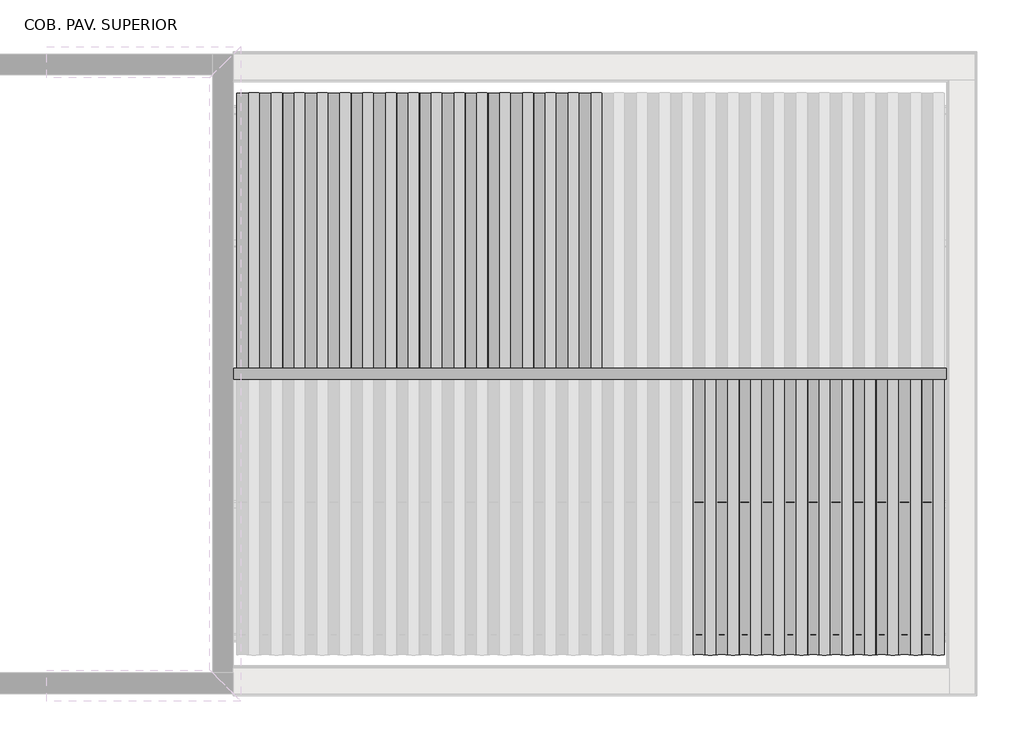
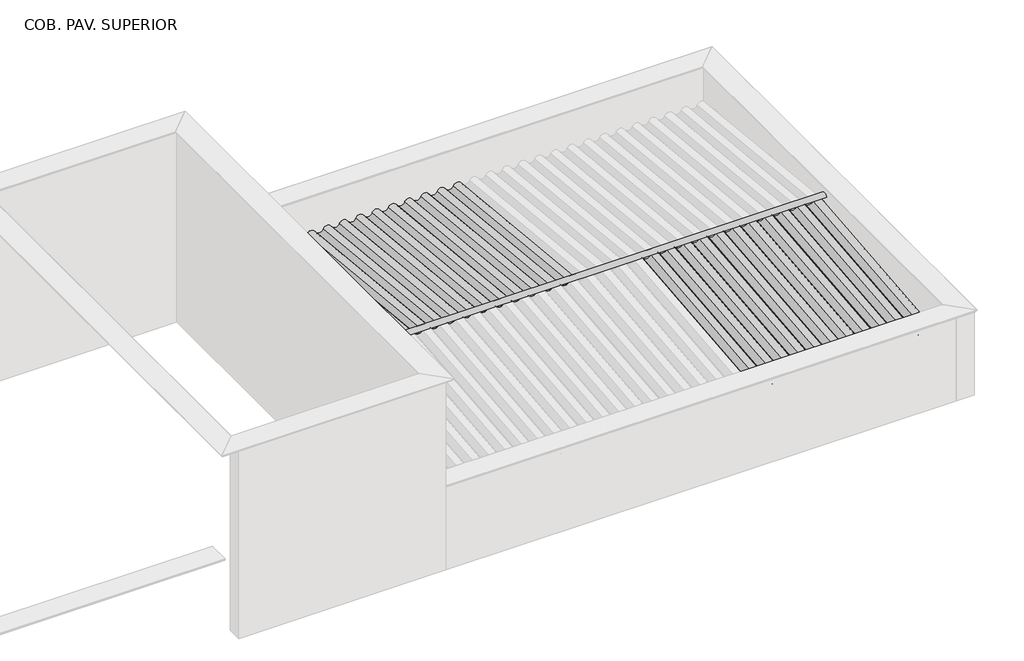
# One storey, part 6 of 7: 35 beams, 6 columns.
"""IFC4 building model written with IfcOpenShell, lengths in millimetres."""

import ifcopenshell
import ifcopenshell.guid

model = None  # the IFC model being written
_history = None  # IfcOwnerHistory: only IFC2X3 demands one
_inside = {}  # id of a spatial element -> (the spatial element, [elements in it])
_under = {}  # id of a project, library or spatial element -> (it, [spatial elements below it])
_declared = {}  # id of a project -> (the project, [libraries it declares])
_typed = {}  # id of a type object -> (the type object, [elements of that type])
_made_of = {}  # id of a material, layer set ... -> (it, [elements and type objects made of it])


def new_model(schema):
    """Start an empty IFC model of exactly this schema.

    Asked for "IFC4X3", IfcOpenShell would pick the latest addendum, in which some entities
    have other attributes; the version numbers below select the first issue.
    IFC2X3 requires an IfcOwnerHistory on every rooted entity: one is made here for all.
    """
    global model, _history
    if schema == "IFC4X3":
        model = ifcopenshell.file(schema_version=(4, 3, 0, 0))
    else:
        model = ifcopenshell.file(schema=schema)
    _inside.clear()
    _under.clear()
    _declared.clear()
    _typed.clear()
    _made_of.clear()
    _history = None
    if model.schema == "IFC2X3":
        org = make("IfcOrganization", Name="unknown")
        user = make(
            "IfcPersonAndOrganization",
            ThePerson=make("IfcPerson", FamilyName="unknown"),
            TheOrganization=org,
        )
        app = make(
            "IfcApplication",
            ApplicationDeveloper=org,
            Version="unknown",
            ApplicationFullName="unknown",
            ApplicationIdentifier="unknown",
        )
        _history = make(
            "IfcOwnerHistory",
            OwningUser=user,
            OwningApplication=app,
            ChangeAction="ADDED",
            CreationDate=0,
        )
    return model


def make(cls, **values):
    """One entity of the class cls with the attributes given. An attribute that is None is left unset."""
    return model.create_entity(
        cls, **{name: value for name, value in values.items() if value is not None}
    )


def rooted(cls, **values):
    """An entity with a GlobalId (a new one), such as an element, a storey or a relation."""
    return make(cls, GlobalId=ifcopenshell.guid.new(), OwnerHistory=_history, **values)


def si_unit(unit_type, name, prefix=None):
    """IfcSIUnit, for example si_unit("LENGTHUNIT", "METRE", prefix="MILLI")."""
    return make("IfcSIUnit", UnitType=unit_type, Prefix=prefix, Name=name)


def assignment(units):
    """IfcUnitAssignment: the units of a project."""
    return None if units is None else make("IfcUnitAssignment", Units=units)


def point(xyz):
    """IfcCartesianPoint."""
    return None if xyz is None else make("IfcCartesianPoint", Coordinates=xyz)


def direction(xyz):
    """IfcDirection."""
    return None if xyz is None else make("IfcDirection", DirectionRatios=xyz)


def frame(location, z_axis=None, x_axis=None):
    """IfcAxis2Placement3D, a coordinate frame: its origin and axes. An axis left out is left unset."""
    return make(
        "IfcAxis2Placement3D",
        Location=point(location),
        Axis=direction(z_axis),
        RefDirection=direction(x_axis),
    )


def frame_2d(location, x_axis=None):
    """IfcAxis2Placement2D, a coordinate frame in the plane: its origin and x axis."""
    return make(
        "IfcAxis2Placement2D", Location=point(location), RefDirection=direction(x_axis)
    )


def origin():
    """The frame at (0, 0, 0) with its axes left unset."""
    return frame((0.0, 0.0, 0.0))


def place(relative_to, where):
    """IfcLocalPlacement: puts the frame where relative to a parent placement (None: the world)."""
    return make(
        "IfcLocalPlacement", PlacementRelTo=relative_to, RelativePlacement=where
    )


def context(
    kind, dimensions, precision=None, world=None, true_north=None, identifier=None
):
    """IfcGeometricRepresentationContext, for example the 3D "Model" context."""
    return make(
        "IfcGeometricRepresentationContext",
        ContextIdentifier=identifier,
        ContextType=kind,
        CoordinateSpaceDimension=dimensions,
        Precision=precision,
        WorldCoordinateSystem=world,
        TrueNorth=true_north,
    )


def project(units=None, contexts=None):
    """IfcProject with its units and contexts."""
    return rooted(
        "IfcProject",
        Name="project",
        RepresentationContexts=contexts,
        UnitsInContext=assignment(units),
    )


def spatial(cls, under=None, at=None, **own):
    """A site, building, storey or space (cls), placed at a placement, below another one or the project."""
    s = rooted(cls, ObjectPlacement=at, **own)
    if under is not None:
        _under.setdefault(under.id(), (under, []))[1].append(s)
    return s


def polyline(points):
    """IfcPolyline through the points."""
    return make("IfcPolyline", Points=[point(p) for p in points])


def circle_curve(where, radius):
    """IfcCircle in the frame where."""
    return make("IfcCircle", Position=where, Radius=radius)


def trimmed(basis, trim1, trim2, sense, master):
    """IfcTrimmedCurve: the piece of a basis curve between two trims."""
    return make(
        "IfcTrimmedCurve",
        BasisCurve=basis,
        Trim1=trim1,
        Trim2=trim2,
        SenseAgreement=sense,
        MasterRepresentation=master,
    )


def segment(curve, same_sense, transition):
    """IfcCompositeCurveSegment."""
    return make(
        "IfcCompositeCurveSegment",
        Transition=transition,
        SameSense=same_sense,
        ParentCurve=curve,
    )


def composite_curve(segments, self_intersect=None):
    """IfcCompositeCurve: segments joined end to end."""
    return make("IfcCompositeCurve", Segments=segments, SelfIntersect=self_intersect)


def outline(outer, holes=None, kind="AREA"):
    """IfcArbitraryClosedProfileDef: a profile drawn as a closed curve; with holes, ...WithVoids."""
    if holes is None:
        return make("IfcArbitraryClosedProfileDef", ProfileType=kind, OuterCurve=outer)
    return make(
        "IfcArbitraryProfileDefWithVoids",
        ProfileType=kind,
        OuterCurve=outer,
        InnerCurves=holes,
    )


def extrude(swept, where, along, depth):
    """IfcExtrudedAreaSolid: the profile swept, set in the frame where, extruded along a direction by depth."""
    return make(
        "IfcExtrudedAreaSolid",
        SweptArea=swept,
        Position=where,
        ExtrudedDirection=direction(along),
        Depth=depth,
    )


def shape(context_of_items, identifier, shape_type, items):
    """IfcShapeRepresentation: the items that make up one representation, for example the "Body"."""
    return make(
        "IfcShapeRepresentation",
        ContextOfItems=context_of_items,
        RepresentationIdentifier=identifier,
        RepresentationType=shape_type,
        Items=items,
    )


def source(mapping_origin, context_of_items, identifier, shape_type, items):
    """IfcRepresentationMap: a shape defined once, which mapped items show again and again."""
    return make(
        "IfcRepresentationMap",
        MappingOrigin=mapping_origin,
        MappedRepresentation=shape(context_of_items, identifier, shape_type, items),
    )


def transform(
    local_origin,
    x_axis=None,
    y_axis=None,
    z_axis=None,
    scale=None,
    scale2=None,
    scale3=None,
    uniform=True,
):
    """IfcCartesianTransformationOperator3D, or its non-uniform kind. x_axis, y_axis, z_axis: its Axis1, 2, 3."""
    if uniform:
        return make(
            "IfcCartesianTransformationOperator3D",
            Axis1=direction(x_axis),
            Axis2=direction(y_axis),
            LocalOrigin=point(local_origin),
            Scale=scale,
            Axis3=direction(z_axis),
        )
    return make(
        "IfcCartesianTransformationOperator3DnonUniform",
        Axis1=direction(x_axis),
        Axis2=direction(y_axis),
        LocalOrigin=point(local_origin),
        Scale=scale,
        Axis3=direction(z_axis),
        Scale2=scale2,
        Scale3=scale3,
    )


def mapped(mapping_source, mapping_target):
    """IfcMappedItem: shows the shape of a source again, moved by a transform."""
    return make(
        "IfcMappedItem", MappingSource=mapping_source, MappingTarget=mapping_target
    )


def made_of(thing, what):
    """Note that an element or type object is made of a material, layer set ...; save() writes the relation."""
    if what is not None:
        _made_of.setdefault(what.id(), (what, []))[1].append(thing)
    return thing


def element(
    cls,
    number,
    at=None,
    inside=None,
    cuts=None,
    type_object=None,
    material=None,
    context=None,
    identifier="Body",
    shape_type=None,
    held_by="IfcProductDefinitionShape",
    body=None,
    shapes=None,
    **own,
):
    """One element of the class cls, such as IfcWall. Its Tag is "e" and its number.

    at: its placement. inside: the storey or other place that contains it. cuts: it is an
    opening in that element (IfcRelVoidsElement). A single representation is given by context,
    identifier, shape_type and body (its items); several are given by shapes. held_by: the class
    of the entity that holds the representations. save() writes the other relations.
    """
    e = rooted(cls, Tag="e%d" % number, ObjectPlacement=at, **own)
    if body is not None:
        shapes = [shape(context, identifier, shape_type, body)]
    if shapes is not None:
        e.Representation = make(held_by, Representations=shapes)
    if inside is not None:
        _inside.setdefault(inside.id(), (inside, []))[1].append(e)
    if cuts is not None:
        rooted(
            "IfcRelVoidsElement", RelatingBuildingElement=cuts, RelatedOpeningElement=e
        )
    if type_object is not None:
        _typed.setdefault(type_object.id(), (type_object, []))[1].append(e)
    return made_of(e, material)


def aggregate(whole, parts):
    """IfcRelAggregates: a whole, such as a stair, and the parts it consists of."""
    return rooted("IfcRelAggregates", RelatingObject=whole, RelatedObjects=parts)


def save(model, path):
    """Write the relations noted so far, then the file.

    IfcRelAggregates (storeys below a building ...), IfcRelContainedInSpatialStructure (elements
    in a storey), IfcRelDefinesByType, IfcRelAssociatesMaterial and IfcRelDeclares: one each for
    every whole, place, type object, material and project.
    """
    for whole, parts in _under.values():
        aggregate(whole, parts)
    for where, things in _inside.values():
        rooted(
            "IfcRelContainedInSpatialStructure",
            RelatedElements=things,
            RelatingStructure=where,
        )
    for kind, things in _typed.values():
        rooted("IfcRelDefinesByType", RelatedObjects=things, RelatingType=kind)
    for what, things in _made_of.values():
        rooted("IfcRelAssociatesMaterial", RelatedObjects=things, RelatingMaterial=what)
    for by, libraries in _declared.values():
        rooted("IfcRelDeclares", RelatingContext=by, RelatedDefinitions=libraries)
    model.write(path)


def cumeeira_telha_ondulada_fibrocimento_a8dbf5af(model_context):
    return source(origin(), model_context, "Body", "SweptSolid", [
        extrude(outline(composite_curve([segment(polyline([(58.3970135, 42.4437972), (53.9055884, 40.2467307)]), True, "CONTINUOUS"), segment(trimmed(circle_curve(frame_2d((-1.6029865, 13.0936483)), 61.7939461), [point((53.9055884, 40.2467307))], [point((-57.1115615, 40.2467307))], True, "CARTESIAN"), True, "CONTINUOUS"), segment(polyline([(-57.1115615, 40.2467307), (-61.6029865, 42.4437972)]), True, "CONTINUOUS"), segment(trimmed(circle_curve(frame_2d((-1.6029865, 13.0936483)), 66.7939461), [point((-61.6029865, 42.4437972))], [point((58.3970135, 42.4437972))], False, "CARTESIAN"), True, "CONTINUOUS")], self_intersect=False)), frame((-3970.0, 0.0, 0.0), z_axis=(1.0, 0.0, 0.0), x_axis=(0.0, 1.0, 0.0)), (0.0, 0.0, 1.0), 7940.0),
    ])


def viga_cumeeira_6x16cm_8fcfcc43(model_context):
    return source(origin(), model_context, "Body", "SweptSolid", [
        extrude(outline(polyline([(3822.5, 30.0), (3822.5, -30.0), (-3822.5, -30.0), (-3822.5, 30.0), (3822.5, 30.0)])), frame((0.0, 0.0, -80.0), z_axis=(0.0, 0.0, 1.0), x_axis=(1.0, 0.0, 0.0)), (0.0, 0.0, 1.0), 160.0),
    ])


def column_d505325c(model_context):
    return source(origin(), model_context, "Body", "SweptSolid", [
        extrude(outline(polyline([(30.0, 80.0), (30.0, -80.0), (-30.0, -80.0), (-30.0, 80.0), (30.0, 80.0)])), frame((0.0, 0.0, 6710.0), z_axis=(0.0, 0.0, 1.0), x_axis=(1.0, 0.0, 0.0)), (0.0, 0.0, 1.0), 750.0),
    ])


def column_4db371bd(model_context):
    return source(origin(), model_context, "Body", "SweptSolid", [
        extrude(outline(polyline([(30.0, 80.0), (30.0, -80.0), (-30.0, -80.0), (-30.0, 80.0), (30.0, 80.0)])), frame((0.0, 0.0, 6710.0), z_axis=(0.0, 0.0, 1.0), x_axis=(1.0, 0.0, 0.0)), (0.0, 0.0, 1.0), 660.0),
    ])


model = new_model("IFC4")

# Units and contexts
model_context = context("Model", 3, world=origin())
ifc_project = project(units=[si_unit("LENGTHUNIT", "METRE", prefix="MILLI")], contexts=[model_context])

# Site, building, storey
site = spatial("IfcSite", under=ifc_project)
building = spatial("IfcBuilding", under=site)
storey = spatial("IfcBuildingStorey", under=building, Name="COB. PAV. SUPERIOR", Elevation=6650.0)

# Beams
placement = place(None, origin())
element("IfcBeam", 1, ObjectType="Madeira de lei : Berço 6x12cm", at=placement, inside=storey, context=model_context, shape_type="SweptSolid", body=[
    extrude(outline(polyline([(5090.718693, -7711.5607799), (5090.718693, -7831.5607799), (3090.718693, -7831.5607799), (3090.718693, -7711.5607799), (5090.718693, -7711.5607799)])), frame((0.0, 0.0, 6650.0), z_axis=(0.0, 0.0, 1.0), x_axis=(1.0, 0.0, 0.0)), (0.0, 0.0, 1.0), 60.0),
])
element("IfcBeam", 2, ObjectType="Madeira de lei : Berço 6x12cm", at=placement, inside=storey, context=model_context, shape_type="SweptSolid", body=[
    extrude(outline(polyline([(7090.718693, -7711.5607799), (7090.718693, -7831.5607799), (5090.718693, -7831.5607799), (5090.718693, -7711.5607799), (7090.718693, -7711.5607799)])), frame((0.0, 0.0, 6650.0), z_axis=(0.0, 0.0, 1.0), x_axis=(1.0, 0.0, 0.0)), (0.0, 0.0, 1.0), 60.0),
])
element("IfcBeam", 3, ObjectType="Madeira de lei : Berço 6x12cm", at=placement, inside=storey, context=model_context, shape_type="SweptSolid", body=[
    extrude(outline(polyline([(5089.7186924, -6319.8711004), (5089.7186924, -6439.8711004), (3089.718693, -6439.8711004), (3089.718693, -6319.8711004), (5089.7186924, -6319.8711004)])), frame((0.0, 0.0, 6650.0), z_axis=(0.0, 0.0, 1.0), x_axis=(1.0, 0.0, 0.0)), (0.0, 0.0, 1.0), 60.0),
])
element("IfcBeam", 4, ObjectType="Madeira de lei : Berço 6x12cm", at=placement, inside=storey, context=model_context, shape_type="SweptSolid", body=[
    extrude(outline(polyline([(7089.7186924, -6319.8711004), (7089.7186924, -6439.8711004), (5089.7186936, -6439.8711004), (5089.7186936, -6319.8711004), (7089.7186924, -6319.8711004)])), frame((0.0, 0.0, 6650.0), z_axis=(0.0, 0.0, 1.0), x_axis=(1.0, 0.0, 0.0)), (0.0, 0.0, 1.0), 60.0),
])
element("IfcBeam", 5, ObjectType="Madeira de lei : Berço 6x12cm", at=placement, inside=storey, context=model_context, shape_type="SweptSolid", body=[
    extrude(outline(polyline([(9089.718693, -9101.268869), (9089.718693, -9221.268869), (7089.718693, -9221.268869), (7089.718693, -9101.268869), (9089.718693, -9101.268869)])), frame((0.0, 0.0, 6650.0), z_axis=(0.0, 0.0, 1.0), x_axis=(1.0, 0.0, 0.0)), (0.0, 0.0, 1.0), 60.0),
])
element("IfcBeam", 6, ObjectType="Madeira de lei : Berço 6x12cm", at=placement, inside=storey, context=model_context, shape_type="SweptSolid", body=[
    extrude(outline(polyline([(10709.718693, -9101.268869), (10709.718693, -9221.268869), (9089.718693, -9221.268869), (9089.718693, -9101.268869), (10709.718693, -9101.268869)])), frame((0.0, 0.0, 6650.0), z_axis=(0.0, 0.0, 1.0), x_axis=(1.0, 0.0, 0.0)), (0.0, 0.0, 1.0), 60.0),
])
cumeeira_telha_ondulada_fibrocimento_shape = cumeeira_telha_ondulada_fibrocimento_a8dbf5af(model_context)
element("IfcBeam", 7, ObjectType="Cumeeira Telha Ondulada : Fibrocimento", at=placement, inside=storey, context=model_context, shape_type="MappedRepresentation", body=[
    mapped(cumeeira_telha_ondulada_fibrocimento_shape, transform((7061.718693, -7771.5607799, 7660.6251229), x_axis=(-1.0, 0.0, 0.0), y_axis=(0.0, -1.0, 0.0), z_axis=(0.0, 0.0, 1.0))),
])
element("IfcBeam", 8, ObjectType="Telha Ondulada : Fibrocimento", at=placement, inside=storey, context=model_context, shape_type="SweptSolid", body=[
    extrude(outline(composite_curve([segment(trimmed(circle_curve(frame_2d((-58.7002978, -53.2060539)), 66.7939461), [point((-29.3501489, 6.7939461))], [point((-29.3501489, -113.2060539))], False, "CARTESIAN"), True, "CONTINUOUS"), segment(polyline([(-29.3501489, -113.2060539), (-31.5472154, -108.7146289)]), True, "CONTINUOUS"), segment(trimmed(circle_curve(frame_2d((-58.7002978, -53.2060539)), 61.7939461), [point((-31.5472154, -108.7146289))], [point((-31.5472154, 2.3025211))], True, "CARTESIAN"), True, "CONTINUOUS"), segment(trimmed(circle_curve(frame_2d((0.0, 66.7939461)), 71.7939461), [point((-31.5472154, 2.3025211))], [point((-31.5472154, 131.2853711))], False, "CARTESIAN"), True, "CONTINUOUS"), segment(polyline([(-31.5472154, 131.2853711), (-29.3501489, 126.7939461)]), True, "CONTINUOUS"), segment(trimmed(circle_curve(frame_2d((0.0, 66.7939461)), 66.7939461), [point((-29.3501489, 126.7939461))], [point((-29.3501489, 6.7939461))], True, "CARTESIAN"), True, "CONTINUOUS")], self_intersect=False)), frame((3256.1156257, -4759.1621575, 7394.5315886), z_axis=(0.0, -0.9950371902099893, 0.09950371902099778), x_axis=(0.0, 0.09950371902099778, 0.9950371902099893)), (0.0, 0.0, 1.0), 3017.2387654),
])
element("IfcBeam", 9, ObjectType="Telha Ondulada : Fibrocimento", at=placement, inside=storey, context=model_context, shape_type="SweptSolid", body=[
    extrude(outline(composite_curve([segment(trimmed(circle_curve(frame_2d((-58.7002978, -53.2060539)), 66.7939461), [point((-29.3501489, 6.7939461))], [point((-29.3501489, -113.2060539))], False, "CARTESIAN"), True, "CONTINUOUS"), segment(polyline([(-29.3501489, -113.2060539), (-31.5472154, -108.7146289)]), True, "CONTINUOUS"), segment(trimmed(circle_curve(frame_2d((-58.7002978, -53.2060539)), 61.7939461), [point((-31.5472154, -108.7146289))], [point((-31.5472154, 2.3025211))], True, "CARTESIAN"), True, "CONTINUOUS"), segment(trimmed(circle_curve(frame_2d((0.0, 66.7939461)), 71.7939461), [point((-31.5472154, 2.3025211))], [point((-31.5472154, 131.2853711))], False, "CARTESIAN"), True, "CONTINUOUS"), segment(polyline([(-31.5472154, 131.2853711), (-29.3501489, 126.7939461)]), True, "CONTINUOUS"), segment(trimmed(circle_curve(frame_2d((0.0, 66.7939461)), 66.7939461), [point((-29.3501489, 126.7939461))], [point((-29.3501489, 6.7939461))], True, "CARTESIAN"), True, "CONTINUOUS")], self_intersect=False)), frame((3500.6156257, -4759.1621575, 7394.5315886), z_axis=(0.0, -0.9950371902099893, 0.09950371902099778), x_axis=(0.0, 0.09950371902099778, 0.9950371902099893)), (0.0, 0.0, 1.0), 3017.2387654),
])
element("IfcBeam", 10, ObjectType="Telha Ondulada : Fibrocimento", at=placement, inside=storey, context=model_context, shape_type="SweptSolid", body=[
    extrude(outline(composite_curve([segment(trimmed(circle_curve(frame_2d((-58.7002978, -53.2060539)), 66.7939461), [point((-29.3501489, 6.7939461))], [point((-29.3501489, -113.2060539))], False, "CARTESIAN"), True, "CONTINUOUS"), segment(polyline([(-29.3501489, -113.2060539), (-31.5472154, -108.7146289)]), True, "CONTINUOUS"), segment(trimmed(circle_curve(frame_2d((-58.7002978, -53.2060539)), 61.7939461), [point((-31.5472154, -108.7146289))], [point((-31.5472154, 2.3025211))], True, "CARTESIAN"), True, "CONTINUOUS"), segment(trimmed(circle_curve(frame_2d((0.0, 66.7939461)), 71.7939461), [point((-31.5472154, 2.3025211))], [point((-31.5472154, 131.2853711))], False, "CARTESIAN"), True, "CONTINUOUS"), segment(polyline([(-31.5472154, 131.2853711), (-29.3501489, 126.7939461)]), True, "CONTINUOUS"), segment(trimmed(circle_curve(frame_2d((0.0, 66.7939461)), 66.7939461), [point((-29.3501489, 126.7939461))], [point((-29.3501489, 6.7939461))], True, "CARTESIAN"), True, "CONTINUOUS")], self_intersect=False)), frame((3745.1156257, -4759.1621575, 7394.5315886), z_axis=(0.0, -0.9950371902099893, 0.09950371902099776), x_axis=(0.0, 0.09950371902099776, 0.9950371902099893)), (0.0, 0.0, 1.0), 3017.2387654),
])
element("IfcBeam", 11, ObjectType="Telha Ondulada : Fibrocimento", at=placement, inside=storey, context=model_context, shape_type="SweptSolid", body=[
    extrude(outline(composite_curve([segment(trimmed(circle_curve(frame_2d((-58.7002978, -53.2060539)), 66.7939461), [point((-29.3501489, 6.7939461))], [point((-29.3501489, -113.2060539))], False, "CARTESIAN"), True, "CONTINUOUS"), segment(polyline([(-29.3501489, -113.2060539), (-31.5472154, -108.7146289)]), True, "CONTINUOUS"), segment(trimmed(circle_curve(frame_2d((-58.7002978, -53.2060539)), 61.7939461), [point((-31.5472154, -108.7146289))], [point((-31.5472154, 2.3025211))], True, "CARTESIAN"), True, "CONTINUOUS"), segment(trimmed(circle_curve(frame_2d((0.0, 66.7939461)), 71.7939461), [point((-31.5472154, 2.3025211))], [point((-31.5472154, 131.2853711))], False, "CARTESIAN"), True, "CONTINUOUS"), segment(polyline([(-31.5472154, 131.2853711), (-29.3501489, 126.7939461)]), True, "CONTINUOUS"), segment(trimmed(circle_curve(frame_2d((0.0, 66.7939461)), 66.7939461), [point((-29.3501489, 126.7939461))], [point((-29.3501489, 6.7939461))], True, "CARTESIAN"), True, "CONTINUOUS")], self_intersect=False)), frame((3989.6156257, -4759.1621575, 7394.5315886), z_axis=(0.0, -0.9950371902099893, 0.09950371902099776), x_axis=(0.0, 0.09950371902099776, 0.9950371902099893)), (0.0, 0.0, 1.0), 3017.2387654),
])
element("IfcBeam", 12, ObjectType="Telha Ondulada : Fibrocimento", at=placement, inside=storey, context=model_context, shape_type="SweptSolid", body=[
    extrude(outline(composite_curve([segment(trimmed(circle_curve(frame_2d((-58.7002978, -53.2060539)), 66.7939461), [point((-29.3501489, 6.7939461))], [point((-29.3501489, -113.2060539))], False, "CARTESIAN"), True, "CONTINUOUS"), segment(polyline([(-29.3501489, -113.2060539), (-31.5472154, -108.7146289)]), True, "CONTINUOUS"), segment(trimmed(circle_curve(frame_2d((-58.7002978, -53.2060539)), 61.7939461), [point((-31.5472154, -108.7146289))], [point((-31.5472154, 2.3025211))], True, "CARTESIAN"), True, "CONTINUOUS"), segment(trimmed(circle_curve(frame_2d((0.0, 66.7939461)), 71.7939461), [point((-31.5472154, 2.3025211))], [point((-31.5472154, 131.2853711))], False, "CARTESIAN"), True, "CONTINUOUS"), segment(polyline([(-31.5472154, 131.2853711), (-29.3501489, 126.7939461)]), True, "CONTINUOUS"), segment(trimmed(circle_curve(frame_2d((0.0, 66.7939461)), 66.7939461), [point((-29.3501489, 126.7939461))], [point((-29.3501489, 6.7939461))], True, "CARTESIAN"), True, "CONTINUOUS")], self_intersect=False)), frame((4234.1156257, -4759.1621575, 7394.5315886), z_axis=(0.0, -0.9950371902099893, 0.09950371902099775), x_axis=(0.0, 0.09950371902099775, 0.9950371902099893)), (0.0, 0.0, 1.0), 3017.2387654),
])
element("IfcBeam", 13, ObjectType="Telha Ondulada : Fibrocimento", at=placement, inside=storey, context=model_context, shape_type="SweptSolid", body=[
    extrude(outline(composite_curve([segment(trimmed(circle_curve(frame_2d((-58.7002978, -53.2060539)), 66.7939461), [point((-29.3501489, 6.7939461))], [point((-29.3501489, -113.2060539))], False, "CARTESIAN"), True, "CONTINUOUS"), segment(polyline([(-29.3501489, -113.2060539), (-31.5472154, -108.7146289)]), True, "CONTINUOUS"), segment(trimmed(circle_curve(frame_2d((-58.7002978, -53.2060539)), 61.7939461), [point((-31.5472154, -108.7146289))], [point((-31.5472154, 2.3025211))], True, "CARTESIAN"), True, "CONTINUOUS"), segment(trimmed(circle_curve(frame_2d((0.0, 66.7939461)), 71.7939461), [point((-31.5472154, 2.3025211))], [point((-31.5472154, 131.2853711))], False, "CARTESIAN"), True, "CONTINUOUS"), segment(polyline([(-31.5472154, 131.2853711), (-29.3501489, 126.7939461)]), True, "CONTINUOUS"), segment(trimmed(circle_curve(frame_2d((0.0, 66.7939461)), 66.7939461), [point((-29.3501489, 126.7939461))], [point((-29.3501489, 6.7939461))], True, "CARTESIAN"), True, "CONTINUOUS")], self_intersect=False)), frame((4478.6156257, -4759.1621575, 7394.5315886), z_axis=(0.0, -0.9950371902099893, 0.09950371902099778), x_axis=(0.0, 0.09950371902099778, 0.9950371902099893)), (0.0, 0.0, 1.0), 3017.2387654),
])
element("IfcBeam", 14, ObjectType="Telha Ondulada : Fibrocimento", at=placement, inside=storey, context=model_context, shape_type="SweptSolid", body=[
    extrude(outline(composite_curve([segment(trimmed(circle_curve(frame_2d((-58.7002978, -53.2060539)), 66.7939461), [point((-29.3501489, 6.7939461))], [point((-29.3501489, -113.2060539))], False, "CARTESIAN"), True, "CONTINUOUS"), segment(polyline([(-29.3501489, -113.2060539), (-31.5472154, -108.7146289)]), True, "CONTINUOUS"), segment(trimmed(circle_curve(frame_2d((-58.7002978, -53.2060539)), 61.7939461), [point((-31.5472154, -108.7146289))], [point((-31.5472154, 2.3025211))], True, "CARTESIAN"), True, "CONTINUOUS"), segment(trimmed(circle_curve(frame_2d((0.0, 66.7939461)), 71.7939461), [point((-31.5472154, 2.3025211))], [point((-31.5472154, 131.2853711))], False, "CARTESIAN"), True, "CONTINUOUS"), segment(polyline([(-31.5472154, 131.2853711), (-29.3501489, 126.7939461)]), True, "CONTINUOUS"), segment(trimmed(circle_curve(frame_2d((0.0, 66.7939461)), 66.7939461), [point((-29.3501489, 126.7939461))], [point((-29.3501489, 6.7939461))], True, "CARTESIAN"), True, "CONTINUOUS")], self_intersect=False)), frame((4723.1156257, -4759.1621575, 7394.5315886), z_axis=(0.0, -0.9950371902099893, 0.09950371902099776), x_axis=(0.0, 0.09950371902099776, 0.9950371902099893)), (0.0, 0.0, 1.0), 3017.2387654),
])
element("IfcBeam", 15, ObjectType="Telha Ondulada : Fibrocimento", at=placement, inside=storey, context=model_context, shape_type="SweptSolid", body=[
    extrude(outline(composite_curve([segment(trimmed(circle_curve(frame_2d((-58.7002978, -53.2060539)), 66.7939461), [point((-29.3501489, 6.7939461))], [point((-29.3501489, -113.2060539))], False, "CARTESIAN"), True, "CONTINUOUS"), segment(polyline([(-29.3501489, -113.2060539), (-31.5472154, -108.7146289)]), True, "CONTINUOUS"), segment(trimmed(circle_curve(frame_2d((-58.7002978, -53.2060539)), 61.7939461), [point((-31.5472154, -108.7146289))], [point((-31.5472154, 2.3025211))], True, "CARTESIAN"), True, "CONTINUOUS"), segment(trimmed(circle_curve(frame_2d((0.0, 66.7939461)), 71.7939461), [point((-31.5472154, 2.3025211))], [point((-31.5472154, 131.2853711))], False, "CARTESIAN"), True, "CONTINUOUS"), segment(polyline([(-31.5472154, 131.2853711), (-29.3501489, 126.7939461)]), True, "CONTINUOUS"), segment(trimmed(circle_curve(frame_2d((0.0, 66.7939461)), 66.7939461), [point((-29.3501489, 126.7939461))], [point((-29.3501489, 6.7939461))], True, "CARTESIAN"), True, "CONTINUOUS")], self_intersect=False)), frame((4967.6156257, -4759.1621575, 7394.5315886), z_axis=(0.0, -0.9950371902099893, 0.09950371902099775), x_axis=(0.0, 0.09950371902099775, 0.9950371902099893)), (0.0, 0.0, 1.0), 3017.2387654),
])
element("IfcBeam", 16, ObjectType="Telha Ondulada : Fibrocimento", at=placement, inside=storey, context=model_context, shape_type="SweptSolid", body=[
    extrude(outline(composite_curve([segment(trimmed(circle_curve(frame_2d((-58.7002978, -53.2060539)), 66.7939461), [point((-29.3501489, 6.7939461))], [point((-29.3501489, -113.2060539))], False, "CARTESIAN"), True, "CONTINUOUS"), segment(polyline([(-29.3501489, -113.2060539), (-31.5472154, -108.7146289)]), True, "CONTINUOUS"), segment(trimmed(circle_curve(frame_2d((-58.7002978, -53.2060539)), 61.7939461), [point((-31.5472154, -108.7146289))], [point((-31.5472154, 2.3025211))], True, "CARTESIAN"), True, "CONTINUOUS"), segment(trimmed(circle_curve(frame_2d((0.0, 66.7939461)), 71.7939461), [point((-31.5472154, 2.3025211))], [point((-31.5472154, 131.2853711))], False, "CARTESIAN"), True, "CONTINUOUS"), segment(polyline([(-31.5472154, 131.2853711), (-29.3501489, 126.7939461)]), True, "CONTINUOUS"), segment(trimmed(circle_curve(frame_2d((0.0, 66.7939461)), 66.7939461), [point((-29.3501489, 126.7939461))], [point((-29.3501489, 6.7939461))], True, "CARTESIAN"), True, "CONTINUOUS")], self_intersect=False)), frame((5212.1156257, -4759.1621575, 7394.5315886), z_axis=(0.0, -0.9950371902099893, 0.09950371902099778), x_axis=(0.0, 0.09950371902099778, 0.9950371902099893)), (0.0, 0.0, 1.0), 3017.2387654),
])
element("IfcBeam", 17, ObjectType="Telha Ondulada : Fibrocimento", at=placement, inside=storey, context=model_context, shape_type="SweptSolid", body=[
    extrude(outline(composite_curve([segment(trimmed(circle_curve(frame_2d((-58.7002978, -53.2060539)), 66.7939461), [point((-29.3501489, 6.7939461))], [point((-29.3501489, -113.2060539))], False, "CARTESIAN"), True, "CONTINUOUS"), segment(polyline([(-29.3501489, -113.2060539), (-31.5472154, -108.7146289)]), True, "CONTINUOUS"), segment(trimmed(circle_curve(frame_2d((-58.7002978, -53.2060539)), 61.7939461), [point((-31.5472154, -108.7146289))], [point((-31.5472154, 2.3025211))], True, "CARTESIAN"), True, "CONTINUOUS"), segment(trimmed(circle_curve(frame_2d((0.0, 66.7939461)), 71.7939461), [point((-31.5472154, 2.3025211))], [point((-31.5472154, 131.2853711))], False, "CARTESIAN"), True, "CONTINUOUS"), segment(polyline([(-31.5472154, 131.2853711), (-29.3501489, 126.7939461)]), True, "CONTINUOUS"), segment(trimmed(circle_curve(frame_2d((0.0, 66.7939461)), 66.7939461), [point((-29.3501489, 126.7939461))], [point((-29.3501489, 6.7939461))], True, "CARTESIAN"), True, "CONTINUOUS")], self_intersect=False)), frame((5456.6156257, -4759.1621575, 7394.5315886), z_axis=(0.0, -0.9950371902099893, 0.09950371902099776), x_axis=(0.0, 0.09950371902099776, 0.9950371902099893)), (0.0, 0.0, 1.0), 3017.2387654),
])
element("IfcBeam", 18, ObjectType="Telha Ondulada : Fibrocimento", at=placement, inside=storey, context=model_context, shape_type="SweptSolid", body=[
    extrude(outline(composite_curve([segment(trimmed(circle_curve(frame_2d((-58.7002978, -53.2060539)), 66.7939461), [point((-29.3501489, 6.7939461))], [point((-29.3501489, -113.2060539))], False, "CARTESIAN"), True, "CONTINUOUS"), segment(polyline([(-29.3501489, -113.2060539), (-31.5472154, -108.7146289)]), True, "CONTINUOUS"), segment(trimmed(circle_curve(frame_2d((-58.7002978, -53.2060539)), 61.7939461), [point((-31.5472154, -108.7146289))], [point((-31.5472154, 2.3025211))], True, "CARTESIAN"), True, "CONTINUOUS"), segment(trimmed(circle_curve(frame_2d((0.0, 66.7939461)), 71.7939461), [point((-31.5472154, 2.3025211))], [point((-31.5472154, 131.2853711))], False, "CARTESIAN"), True, "CONTINUOUS"), segment(polyline([(-31.5472154, 131.2853711), (-29.3501489, 126.7939461)]), True, "CONTINUOUS"), segment(trimmed(circle_curve(frame_2d((0.0, 66.7939461)), 66.7939461), [point((-29.3501489, 126.7939461))], [point((-29.3501489, 6.7939461))], True, "CARTESIAN"), True, "CONTINUOUS")], self_intersect=False)), frame((5701.1156257, -4759.1621575, 7394.5315886), z_axis=(0.0, -0.9950371902099893, 0.09950371902099776), x_axis=(0.0, 0.09950371902099776, 0.9950371902099893)), (0.0, 0.0, 1.0), 3017.2387654),
])
element("IfcBeam", 19, ObjectType="Telha Ondulada : Fibrocimento", at=placement, inside=storey, context=model_context, shape_type="SweptSolid", body=[
    extrude(outline(composite_curve([segment(trimmed(circle_curve(frame_2d((-58.7002978, -53.2060539)), 66.7939461), [point((-29.3501489, 6.7939461))], [point((-29.3501489, -113.2060539))], False, "CARTESIAN"), True, "CONTINUOUS"), segment(polyline([(-29.3501489, -113.2060539), (-31.5472154, -108.7146289)]), True, "CONTINUOUS"), segment(trimmed(circle_curve(frame_2d((-58.7002978, -53.2060539)), 61.7939461), [point((-31.5472154, -108.7146289))], [point((-31.5472154, 2.3025211))], True, "CARTESIAN"), True, "CONTINUOUS"), segment(trimmed(circle_curve(frame_2d((0.0, 66.7939461)), 71.7939461), [point((-31.5472154, 2.3025211))], [point((-31.5472154, 131.2853711))], False, "CARTESIAN"), True, "CONTINUOUS"), segment(polyline([(-31.5472154, 131.2853711), (-29.3501489, 126.7939461)]), True, "CONTINUOUS"), segment(trimmed(circle_curve(frame_2d((0.0, 66.7939461)), 66.7939461), [point((-29.3501489, 126.7939461))], [point((-29.3501489, 6.7939461))], True, "CARTESIAN"), True, "CONTINUOUS")], self_intersect=False)), frame((5945.6156257, -4759.1621575, 7394.5315886), z_axis=(0.0, -0.9950371902099893, 0.09950371902099778), x_axis=(0.0, 0.09950371902099778, 0.9950371902099893)), (0.0, 0.0, 1.0), 3017.2387654),
])
element("IfcBeam", 20, ObjectType="Telha Ondulada : Fibrocimento", at=placement, inside=storey, context=model_context, shape_type="SweptSolid", body=[
    extrude(outline(composite_curve([segment(trimmed(circle_curve(frame_2d((-58.7002978, -53.2060539)), 66.7939461), [point((-29.3501489, 6.7939461))], [point((-29.3501489, -113.2060539))], False, "CARTESIAN"), True, "CONTINUOUS"), segment(polyline([(-29.3501489, -113.2060539), (-31.5472154, -108.7146289)]), True, "CONTINUOUS"), segment(trimmed(circle_curve(frame_2d((-58.7002978, -53.2060539)), 61.7939461), [point((-31.5472154, -108.7146289))], [point((-31.5472154, 2.3025211))], True, "CARTESIAN"), True, "CONTINUOUS"), segment(trimmed(circle_curve(frame_2d((0.0, 66.7939461)), 71.7939461), [point((-31.5472154, 2.3025211))], [point((-31.5472154, 131.2853711))], False, "CARTESIAN"), True, "CONTINUOUS"), segment(polyline([(-31.5472154, 131.2853711), (-29.3501489, 126.7939461)]), True, "CONTINUOUS"), segment(trimmed(circle_curve(frame_2d((0.0, 66.7939461)), 66.7939461), [point((-29.3501489, 126.7939461))], [point((-29.3501489, 6.7939461))], True, "CARTESIAN"), True, "CONTINUOUS")], self_intersect=False)), frame((6190.1156257, -4759.1621575, 7394.5315886), z_axis=(0.0, -0.9950371902099893, 0.09950371902099778), x_axis=(0.0, 0.09950371902099778, 0.9950371902099893)), (0.0, 0.0, 1.0), 3017.2387654),
])
element("IfcBeam", 21, ObjectType="Telha Ondulada : Fibrocimento", at=placement, inside=storey, context=model_context, shape_type="SweptSolid", body=[
    extrude(outline(composite_curve([segment(trimmed(circle_curve(frame_2d((-58.7002978, -53.2060539)), 66.7939461), [point((-29.3501489, 6.7939461))], [point((-29.3501489, -113.2060539))], False, "CARTESIAN"), True, "CONTINUOUS"), segment(polyline([(-29.3501489, -113.2060539), (-31.5472154, -108.7146289)]), True, "CONTINUOUS"), segment(trimmed(circle_curve(frame_2d((-58.7002978, -53.2060539)), 61.7939461), [point((-31.5472154, -108.7146289))], [point((-31.5472154, 2.3025211))], True, "CARTESIAN"), True, "CONTINUOUS"), segment(trimmed(circle_curve(frame_2d((0.0, 66.7939461)), 71.7939461), [point((-31.5472154, 2.3025211))], [point((-31.5472154, 131.2853711))], False, "CARTESIAN"), True, "CONTINUOUS"), segment(polyline([(-31.5472154, 131.2853711), (-29.3501489, 126.7939461)]), True, "CONTINUOUS"), segment(trimmed(circle_curve(frame_2d((0.0, 66.7939461)), 66.7939461), [point((-29.3501489, 126.7939461))], [point((-29.3501489, 6.7939461))], True, "CARTESIAN"), True, "CONTINUOUS")], self_intersect=False)), frame((6434.6156257, -4759.1621575, 7394.5315886), z_axis=(0.0, -0.9950371902099893, 0.09950371902099776), x_axis=(0.0, 0.09950371902099776, 0.9950371902099893)), (0.0, 0.0, 1.0), 3017.2387654),
])
element("IfcBeam", 22, ObjectType="Telha Ondulada : Fibrocimento", at=placement, inside=storey, context=model_context, shape_type="SweptSolid", body=[
    extrude(outline(composite_curve([segment(trimmed(circle_curve(frame_2d((-58.7002978, -53.2060539)), 66.7939461), [point((-29.3501489, 6.7939461))], [point((-29.3501489, -113.2060539))], False, "CARTESIAN"), True, "CONTINUOUS"), segment(polyline([(-29.3501489, -113.2060539), (-31.5472154, -108.7146289)]), True, "CONTINUOUS"), segment(trimmed(circle_curve(frame_2d((-58.7002978, -53.2060539)), 61.7939461), [point((-31.5472154, -108.7146289))], [point((-31.5472154, 2.3025211))], True, "CARTESIAN"), True, "CONTINUOUS"), segment(trimmed(circle_curve(frame_2d((0.0, 66.7939461)), 71.7939461), [point((-31.5472154, 2.3025211))], [point((-31.5472154, 131.2853711))], False, "CARTESIAN"), True, "CONTINUOUS"), segment(polyline([(-31.5472154, 131.2853711), (-29.3501489, 126.7939461)]), True, "CONTINUOUS"), segment(trimmed(circle_curve(frame_2d((0.0, 66.7939461)), 66.7939461), [point((-29.3501489, 126.7939461))], [point((-29.3501489, 6.7939461))], True, "CARTESIAN"), True, "CONTINUOUS")], self_intersect=False)), frame((6679.1156257, -4759.1621575, 7394.5315886), z_axis=(0.0, -0.9950371902099893, 0.09950371902099776), x_axis=(0.0, 0.09950371902099776, 0.9950371902099893)), (0.0, 0.0, 1.0), 3017.2387654),
])
element("IfcBeam", 23, ObjectType="Telha Ondulada : Fibrocimento", at=placement, inside=storey, context=model_context, shape_type="SweptSolid", body=[
    extrude(outline(composite_curve([segment(trimmed(circle_curve(frame_2d((-58.7002978, -53.2060539)), 66.7939461), [point((-29.3501489, 6.7939461))], [point((-29.3501489, -113.2060539))], False, "CARTESIAN"), True, "CONTINUOUS"), segment(polyline([(-29.3501489, -113.2060539), (-31.5472154, -108.7146289)]), True, "CONTINUOUS"), segment(trimmed(circle_curve(frame_2d((-58.7002978, -53.2060539)), 61.7939461), [point((-31.5472154, -108.7146289))], [point((-31.5472154, 2.3025211))], True, "CARTESIAN"), True, "CONTINUOUS"), segment(trimmed(circle_curve(frame_2d((0.0, 66.7939461)), 71.7939461), [point((-31.5472154, 2.3025211))], [point((-31.5472154, 131.2853711))], False, "CARTESIAN"), True, "CONTINUOUS"), segment(polyline([(-31.5472154, 131.2853711), (-29.3501489, 126.7939461)]), True, "CONTINUOUS"), segment(trimmed(circle_curve(frame_2d((0.0, 66.7939461)), 66.7939461), [point((-29.3501489, 126.7939461))], [point((-29.3501489, 6.7939461))], True, "CARTESIAN"), True, "CONTINUOUS")], self_intersect=False)), frame((6923.6156257, -4759.1621575, 7394.5315886), z_axis=(0.0, -0.9950371902099893, 0.09950371902099775), x_axis=(0.0, 0.09950371902099775, 0.9950371902099893)), (0.0, 0.0, 1.0), 3017.2387654),
])
element("IfcBeam", 24, ObjectType="Telha Ondulada : Fibrocimento", at=placement, inside=storey, context=model_context, shape_type="SweptSolid", body=[
    extrude(outline(composite_curve([segment(trimmed(circle_curve(frame_2d((0.0, 66.7939461)), 66.7939461), [point((29.3501489, 6.7939461))], [point((29.3501489, 126.7939461))], True, "CARTESIAN"), True, "CONTINUOUS"), segment(polyline([(29.3501489, 126.7939461), (31.5472154, 131.2853711)]), True, "CONTINUOUS"), segment(trimmed(circle_curve(frame_2d((0.0, 66.7939461)), 71.7939461), [point((31.5472154, 131.2853711))], [point((31.5472154, 2.3025211))], False, "CARTESIAN"), True, "CONTINUOUS"), segment(trimmed(circle_curve(frame_2d((58.7002978, -53.2060539)), 61.7939461), [point((31.5472154, 2.3025211))], [point((31.5472154, -108.7146289))], True, "CARTESIAN"), True, "CONTINUOUS"), segment(polyline([(31.5472154, -108.7146289), (29.3501489, -113.2060539)]), True, "CONTINUOUS"), segment(trimmed(circle_curve(frame_2d((58.7002978, -53.2060539)), 66.7939461), [point((29.3501489, -113.2060539))], [point((29.3501489, 6.7939461))], False, "CARTESIAN"), True, "CONTINUOUS")], self_intersect=False)), frame((8146.1156257, -10781.9594023, 7394.5315886), z_axis=(0.0, 0.9950371902099894, 0.09950371902099751), x_axis=(0.0, 0.09950371902099751, -0.9950371902099894)), (0.0, 0.0, 1.0), 3017.2387654),
])
element("IfcBeam", 25, ObjectType="Telha Ondulada : Fibrocimento", at=placement, inside=storey, context=model_context, shape_type="SweptSolid", body=[
    extrude(outline(composite_curve([segment(trimmed(circle_curve(frame_2d((0.0, 66.7939461)), 66.7939461), [point((29.3501489, 6.7939461))], [point((29.3501489, 126.7939461))], True, "CARTESIAN"), True, "CONTINUOUS"), segment(polyline([(29.3501489, 126.7939461), (31.5472154, 131.2853711)]), True, "CONTINUOUS"), segment(trimmed(circle_curve(frame_2d((0.0, 66.7939461)), 71.7939461), [point((31.5472154, 131.2853711))], [point((31.5472154, 2.3025211))], False, "CARTESIAN"), True, "CONTINUOUS"), segment(trimmed(circle_curve(frame_2d((58.7002978, -53.2060539)), 61.7939461), [point((31.5472154, 2.3025211))], [point((31.5472154, -108.7146289))], True, "CARTESIAN"), True, "CONTINUOUS"), segment(polyline([(31.5472154, -108.7146289), (29.3501489, -113.2060539)]), True, "CONTINUOUS"), segment(trimmed(circle_curve(frame_2d((58.7002978, -53.2060539)), 66.7939461), [point((29.3501489, -113.2060539))], [point((29.3501489, 6.7939461))], False, "CARTESIAN"), True, "CONTINUOUS")], self_intersect=False)), frame((8390.6156257, -10781.9594023, 7394.5315886), z_axis=(0.0, 0.9950371902099894, 0.09950371902099751), x_axis=(0.0, 0.09950371902099751, -0.9950371902099894)), (0.0, 0.0, 1.0), 3017.2387654),
])
element("IfcBeam", 26, ObjectType="Telha Ondulada : Fibrocimento", at=placement, inside=storey, context=model_context, shape_type="SweptSolid", body=[
    extrude(outline(composite_curve([segment(trimmed(circle_curve(frame_2d((0.0, 66.7939461)), 66.7939461), [point((29.3501489, 6.7939461))], [point((29.3501489, 126.7939461))], True, "CARTESIAN"), True, "CONTINUOUS"), segment(polyline([(29.3501489, 126.7939461), (31.5472154, 131.2853711)]), True, "CONTINUOUS"), segment(trimmed(circle_curve(frame_2d((0.0, 66.7939461)), 71.7939461), [point((31.5472154, 131.2853711))], [point((31.5472154, 2.3025211))], False, "CARTESIAN"), True, "CONTINUOUS"), segment(trimmed(circle_curve(frame_2d((58.7002978, -53.2060539)), 61.7939461), [point((31.5472154, 2.3025211))], [point((31.5472154, -108.7146289))], True, "CARTESIAN"), True, "CONTINUOUS"), segment(polyline([(31.5472154, -108.7146289), (29.3501489, -113.2060539)]), True, "CONTINUOUS"), segment(trimmed(circle_curve(frame_2d((58.7002978, -53.2060539)), 66.7939461), [point((29.3501489, -113.2060539))], [point((29.3501489, 6.7939461))], False, "CARTESIAN"), True, "CONTINUOUS")], self_intersect=False)), frame((8635.1156257, -10781.9594023, 7394.5315886), z_axis=(0.0, 0.9950371902099894, 0.09950371902099747), x_axis=(0.0, 0.09950371902099747, -0.9950371902099894)), (0.0, 0.0, 1.0), 3017.2387654),
])
element("IfcBeam", 27, ObjectType="Telha Ondulada : Fibrocimento", at=placement, inside=storey, context=model_context, shape_type="SweptSolid", body=[
    extrude(outline(composite_curve([segment(trimmed(circle_curve(frame_2d((0.0, 66.7939461)), 66.7939461), [point((29.3501489, 6.7939461))], [point((29.3501489, 126.7939461))], True, "CARTESIAN"), True, "CONTINUOUS"), segment(polyline([(29.3501489, 126.7939461), (31.5472154, 131.2853711)]), True, "CONTINUOUS"), segment(trimmed(circle_curve(frame_2d((0.0, 66.7939461)), 71.7939461), [point((31.5472154, 131.2853711))], [point((31.5472154, 2.3025211))], False, "CARTESIAN"), True, "CONTINUOUS"), segment(trimmed(circle_curve(frame_2d((58.7002978, -53.2060539)), 61.7939461), [point((31.5472154, 2.3025211))], [point((31.5472154, -108.7146289))], True, "CARTESIAN"), True, "CONTINUOUS"), segment(polyline([(31.5472154, -108.7146289), (29.3501489, -113.2060539)]), True, "CONTINUOUS"), segment(trimmed(circle_curve(frame_2d((58.7002978, -53.2060539)), 66.7939461), [point((29.3501489, -113.2060539))], [point((29.3501489, 6.7939461))], False, "CARTESIAN"), True, "CONTINUOUS")], self_intersect=False)), frame((8879.6156257, -10781.9594023, 7394.5315886), z_axis=(0.0, 0.9950371902099894, 0.09950371902099747), x_axis=(0.0, 0.09950371902099747, -0.9950371902099894)), (0.0, 0.0, 1.0), 3017.2387654),
])
element("IfcBeam", 28, ObjectType="Telha Ondulada : Fibrocimento", at=placement, inside=storey, context=model_context, shape_type="SweptSolid", body=[
    extrude(outline(composite_curve([segment(trimmed(circle_curve(frame_2d((0.0, 66.7939461)), 66.7939461), [point((29.3501489, 6.7939461))], [point((29.3501489, 126.7939461))], True, "CARTESIAN"), True, "CONTINUOUS"), segment(polyline([(29.3501489, 126.7939461), (31.5472154, 131.2853711)]), True, "CONTINUOUS"), segment(trimmed(circle_curve(frame_2d((0.0, 66.7939461)), 71.7939461), [point((31.5472154, 131.2853711))], [point((31.5472154, 2.3025211))], False, "CARTESIAN"), True, "CONTINUOUS"), segment(trimmed(circle_curve(frame_2d((58.7002978, -53.2060539)), 61.7939461), [point((31.5472154, 2.3025211))], [point((31.5472154, -108.7146289))], True, "CARTESIAN"), True, "CONTINUOUS"), segment(polyline([(31.5472154, -108.7146289), (29.3501489, -113.2060539)]), True, "CONTINUOUS"), segment(trimmed(circle_curve(frame_2d((58.7002978, -53.2060539)), 66.7939461), [point((29.3501489, -113.2060539))], [point((29.3501489, 6.7939461))], False, "CARTESIAN"), True, "CONTINUOUS")], self_intersect=False)), frame((9124.1156257, -10781.9594023, 7394.5315886), z_axis=(0.0, 0.9950371902099894, 0.09950371902099744), x_axis=(0.0, 0.09950371902099744, -0.9950371902099894)), (0.0, 0.0, 1.0), 3017.2387654),
])
element("IfcBeam", 29, ObjectType="Telha Ondulada : Fibrocimento", at=placement, inside=storey, context=model_context, shape_type="SweptSolid", body=[
    extrude(outline(composite_curve([segment(trimmed(circle_curve(frame_2d((0.0, 66.7939461)), 66.7939461), [point((29.3501489, 6.7939461))], [point((29.3501489, 126.7939461))], True, "CARTESIAN"), True, "CONTINUOUS"), segment(polyline([(29.3501489, 126.7939461), (31.5472154, 131.2853711)]), True, "CONTINUOUS"), segment(trimmed(circle_curve(frame_2d((0.0, 66.7939461)), 71.7939461), [point((31.5472154, 131.2853711))], [point((31.5472154, 2.3025211))], False, "CARTESIAN"), True, "CONTINUOUS"), segment(trimmed(circle_curve(frame_2d((58.7002978, -53.2060539)), 61.7939461), [point((31.5472154, 2.3025211))], [point((31.5472154, -108.7146289))], True, "CARTESIAN"), True, "CONTINUOUS"), segment(polyline([(31.5472154, -108.7146289), (29.3501489, -113.2060539)]), True, "CONTINUOUS"), segment(trimmed(circle_curve(frame_2d((58.7002978, -53.2060539)), 66.7939461), [point((29.3501489, -113.2060539))], [point((29.3501489, 6.7939461))], False, "CARTESIAN"), True, "CONTINUOUS")], self_intersect=False)), frame((9368.6156257, -10781.9594023, 7394.5315886), z_axis=(0.0, 0.9950371902099894, 0.09950371902099744), x_axis=(0.0, 0.09950371902099744, -0.9950371902099894)), (0.0, 0.0, 1.0), 3017.2387654),
])
element("IfcBeam", 30, ObjectType="Telha Ondulada : Fibrocimento", at=placement, inside=storey, context=model_context, shape_type="SweptSolid", body=[
    extrude(outline(composite_curve([segment(trimmed(circle_curve(frame_2d((0.0, 66.7939461)), 66.7939461), [point((29.3501489, 6.7939461))], [point((29.3501489, 126.7939461))], True, "CARTESIAN"), True, "CONTINUOUS"), segment(polyline([(29.3501489, 126.7939461), (31.5472154, 131.2853711)]), True, "CONTINUOUS"), segment(trimmed(circle_curve(frame_2d((0.0, 66.7939461)), 71.7939461), [point((31.5472154, 131.2853711))], [point((31.5472154, 2.3025211))], False, "CARTESIAN"), True, "CONTINUOUS"), segment(trimmed(circle_curve(frame_2d((58.7002978, -53.2060539)), 61.7939461), [point((31.5472154, 2.3025211))], [point((31.5472154, -108.7146289))], True, "CARTESIAN"), True, "CONTINUOUS"), segment(polyline([(31.5472154, -108.7146289), (29.3501489, -113.2060539)]), True, "CONTINUOUS"), segment(trimmed(circle_curve(frame_2d((58.7002978, -53.2060539)), 66.7939461), [point((29.3501489, -113.2060539))], [point((29.3501489, 6.7939461))], False, "CARTESIAN"), True, "CONTINUOUS")], self_intersect=False)), frame((9613.1156257, -10781.9594023, 7394.5315886), z_axis=(0.0, 0.9950371902099894, 0.09950371902099751), x_axis=(0.0, 0.09950371902099751, -0.9950371902099894)), (0.0, 0.0, 1.0), 3017.2387654),
])
element("IfcBeam", 31, ObjectType="Telha Ondulada : Fibrocimento", at=placement, inside=storey, context=model_context, shape_type="SweptSolid", body=[
    extrude(outline(composite_curve([segment(trimmed(circle_curve(frame_2d((0.0, 66.7939461)), 66.7939461), [point((29.3501489, 6.7939461))], [point((29.3501489, 126.7939461))], True, "CARTESIAN"), True, "CONTINUOUS"), segment(polyline([(29.3501489, 126.7939461), (31.5472154, 131.2853711)]), True, "CONTINUOUS"), segment(trimmed(circle_curve(frame_2d((0.0, 66.7939461)), 71.7939461), [point((31.5472154, 131.2853711))], [point((31.5472154, 2.3025211))], False, "CARTESIAN"), True, "CONTINUOUS"), segment(trimmed(circle_curve(frame_2d((58.7002978, -53.2060539)), 61.7939461), [point((31.5472154, 2.3025211))], [point((31.5472154, -108.7146289))], True, "CARTESIAN"), True, "CONTINUOUS"), segment(polyline([(31.5472154, -108.7146289), (29.3501489, -113.2060539)]), True, "CONTINUOUS"), segment(trimmed(circle_curve(frame_2d((58.7002978, -53.2060539)), 66.7939461), [point((29.3501489, -113.2060539))], [point((29.3501489, 6.7939461))], False, "CARTESIAN"), True, "CONTINUOUS")], self_intersect=False)), frame((9857.6156257, -10781.9594023, 7394.5315886), z_axis=(0.0, 0.9950371902099894, 0.09950371902099751), x_axis=(0.0, 0.09950371902099751, -0.9950371902099894)), (0.0, 0.0, 1.0), 3017.2387654),
])
element("IfcBeam", 32, ObjectType="Telha Ondulada : Fibrocimento", at=placement, inside=storey, context=model_context, shape_type="SweptSolid", body=[
    extrude(outline(composite_curve([segment(trimmed(circle_curve(frame_2d((0.0, 66.7939461)), 66.7939461), [point((29.3501489, 6.7939461))], [point((29.3501489, 126.7939461))], True, "CARTESIAN"), True, "CONTINUOUS"), segment(polyline([(29.3501489, 126.7939461), (31.5472154, 131.2853711)]), True, "CONTINUOUS"), segment(trimmed(circle_curve(frame_2d((0.0, 66.7939461)), 71.7939461), [point((31.5472154, 131.2853711))], [point((31.5472154, 2.3025211))], False, "CARTESIAN"), True, "CONTINUOUS"), segment(trimmed(circle_curve(frame_2d((58.7002978, -53.2060539)), 61.7939461), [point((31.5472154, 2.3025211))], [point((31.5472154, -108.7146289))], True, "CARTESIAN"), True, "CONTINUOUS"), segment(polyline([(31.5472154, -108.7146289), (29.3501489, -113.2060539)]), True, "CONTINUOUS"), segment(trimmed(circle_curve(frame_2d((58.7002978, -53.2060539)), 66.7939461), [point((29.3501489, -113.2060539))], [point((29.3501489, 6.7939461))], False, "CARTESIAN"), True, "CONTINUOUS")], self_intersect=False)), frame((10102.1156257, -10781.9594023, 7394.5315886), z_axis=(0.0, 0.9950371902099894, 0.09950371902099747), x_axis=(0.0, 0.09950371902099747, -0.9950371902099894)), (0.0, 0.0, 1.0), 3017.2387654),
])
element("IfcBeam", 33, ObjectType="Telha Ondulada : Fibrocimento", at=placement, inside=storey, context=model_context, shape_type="SweptSolid", body=[
    extrude(outline(composite_curve([segment(trimmed(circle_curve(frame_2d((0.0, 66.7939461)), 66.7939461), [point((29.3501489, 6.7939461))], [point((29.3501489, 126.7939461))], True, "CARTESIAN"), True, "CONTINUOUS"), segment(polyline([(29.3501489, 126.7939461), (31.5472154, 131.2853711)]), True, "CONTINUOUS"), segment(trimmed(circle_curve(frame_2d((0.0, 66.7939461)), 71.7939461), [point((31.5472154, 131.2853711))], [point((31.5472154, 2.3025211))], False, "CARTESIAN"), True, "CONTINUOUS"), segment(trimmed(circle_curve(frame_2d((58.7002978, -53.2060539)), 61.7939461), [point((31.5472154, 2.3025211))], [point((31.5472154, -108.7146289))], True, "CARTESIAN"), True, "CONTINUOUS"), segment(polyline([(31.5472154, -108.7146289), (29.3501489, -113.2060539)]), True, "CONTINUOUS"), segment(trimmed(circle_curve(frame_2d((58.7002978, -53.2060539)), 66.7939461), [point((29.3501489, -113.2060539))], [point((29.3501489, 6.7939461))], False, "CARTESIAN"), True, "CONTINUOUS")], self_intersect=False)), frame((10346.6156257, -10781.9594023, 7394.5315886), z_axis=(0.0, 0.9950371902099894, 0.09950371902099747), x_axis=(0.0, 0.09950371902099747, -0.9950371902099894)), (0.0, 0.0, 1.0), 3017.2387654),
])
element("IfcBeam", 34, ObjectType="Telha Ondulada : Fibrocimento", at=placement, inside=storey, context=model_context, shape_type="SweptSolid", body=[
    extrude(outline(composite_curve([segment(trimmed(circle_curve(frame_2d((0.0, 66.7939461)), 66.7939461), [point((29.3501489, 6.7939461))], [point((29.3501489, 126.7939461))], True, "CARTESIAN"), True, "CONTINUOUS"), segment(polyline([(29.3501489, 126.7939461), (31.5472154, 131.2853711)]), True, "CONTINUOUS"), segment(trimmed(circle_curve(frame_2d((0.0, 66.7939461)), 71.7939461), [point((31.5472154, 131.2853711))], [point((31.5472154, 2.3025211))], False, "CARTESIAN"), True, "CONTINUOUS"), segment(trimmed(circle_curve(frame_2d((58.7002978, -53.2060539)), 61.7939461), [point((31.5472154, 2.3025211))], [point((31.5472154, -108.7146289))], True, "CARTESIAN"), True, "CONTINUOUS"), segment(polyline([(31.5472154, -108.7146289), (29.3501489, -113.2060539)]), True, "CONTINUOUS"), segment(trimmed(circle_curve(frame_2d((58.7002978, -53.2060539)), 66.7939461), [point((29.3501489, -113.2060539))], [point((29.3501489, 6.7939461))], False, "CARTESIAN"), True, "CONTINUOUS")], self_intersect=False)), frame((10591.1156257, -10781.9594023, 7394.5315886), z_axis=(0.0, 0.9950371902099894, 0.09950371902099744), x_axis=(0.0, 0.09950371902099744, -0.9950371902099894)), (0.0, 0.0, 1.0), 3017.2387654),
])
viga_cumeeira_6x16cm_shape = viga_cumeeira_6x16cm_8fcfcc43(model_context)
element("IfcBeam", 35, ObjectType="Madeira de lei : Viga Cumeeira 6x16cm", at=placement, inside=storey, context=model_context, shape_type="MappedRepresentation", body=[
    mapped(viga_cumeeira_6x16cm_shape, transform((6913.218693, -7771.5607799, 7540.0), x_axis=(1.0, 0.0, 0.0), y_axis=(0.0, 1.0, 0.0), z_axis=(0.0, 0.0, 1.0))),
])

# Columns
column_shape = column_d505325c(model_context)
element("IfcColumn", 36, ObjectType="Madeira de lei-Coluna : Pontalete 6X16cm", at=placement, inside=storey, context=model_context, shape_type="MappedRepresentation", body=[
    mapped(column_shape, transform((4090.718693, -7771.5607799, 0.0), x_axis=(0.0, 1.0, 0.0), y_axis=(-1.0, 0.0, 0.0), z_axis=(0.0, 0.0, 1.0))),
])
element("IfcColumn", 37, ObjectType="Madeira de lei-Coluna : Pontalete 6X16cm", at=placement, inside=storey, context=model_context, shape_type="MappedRepresentation", body=[
    mapped(column_shape, transform((6090.718693, -7771.5607799, 0.0), x_axis=(0.0, 1.0, 0.0), y_axis=(-1.0, 0.0, 0.0), z_axis=(0.0, 0.0, 1.0))),
])
column_2_shape = column_4db371bd(model_context)
element("IfcColumn", 38, ObjectType="Madeira de lei-Coluna : Pontalete 6X16cm", at=placement, inside=storey, context=model_context, shape_type="MappedRepresentation", body=[
    mapped(column_2_shape, transform((4089.718693, -6379.8711004, 0.0), x_axis=(0.0, 1.0, 0.0), y_axis=(-1.0, 0.0, 0.0), z_axis=(0.0, 0.0, 1.0))),
])
element("IfcColumn", 39, ObjectType="Madeira de lei-Coluna : Pontalete 6X16cm", at=placement, inside=storey, context=model_context, shape_type="MappedRepresentation", body=[
    mapped(column_2_shape, transform((6089.718693, -6379.8711004, 0.0), x_axis=(0.0, 1.0, 0.0), y_axis=(-1.0, 0.0, 0.0), z_axis=(0.0, 0.0, 1.0))),
])
element("IfcColumn", 40, ObjectType="Madeira de lei-Coluna : Pontalete 6X16cm", at=placement, inside=storey, context=model_context, shape_type="MappedRepresentation", body=[
    mapped(column_2_shape, transform((8089.718693, -9161.268869, 0.0), x_axis=(0.0, 1.0, 0.0), y_axis=(-1.0, 0.0, 0.0), z_axis=(0.0, 0.0, 1.0))),
])
element("IfcColumn", 41, ObjectType="Madeira de lei-Coluna : Pontalete 6X16cm", at=placement, inside=storey, context=model_context, shape_type="MappedRepresentation", body=[
    mapped(column_2_shape, transform((10089.718693, -9161.268869, 0.0), x_axis=(0.0, 1.0, 0.0), y_axis=(-1.0, 0.0, 0.0), z_axis=(0.0, 0.0, 1.0))),
])

save(model, "model.ifc")

# Revit data of these elements
# Type "Madeira de lei : Berço 6x12cm"
#   A = 0.02 m²
#   Length [instance default] = 1.524 m
#   b = 0.06 m
#   d = 0.12 m
#   Structural Material [instance default] = none
#   Assembly Code = ""
# Type "Cumeeira Telha Ondulada : Fibrocimento"
#   Cost = 5
#   Length [instance default] = 1.524 m
#   b = 0.07 m
#   h = 0.16 m
#   Structural Material = .TELHA DE FIBROCIMENTO
#   Assembly Code = ""
# Type "Telha Ondulada : Fibrocimento"
#   Description = "TELHA ONDULADA FIBROCIMENTO"
#   Cost = 5
#   Length [instance default] = 1.524 m
#   b = 0.07 m
#   h = 0.16 m
#   Structural Material = .TELHA DE FIBROCIMENTO
#   Assembly Code = ""
# Type "Madeira de lei : Viga Cumeeira 6x16cm"
#   A = 0.02 m²
#   Length [instance default] = 1.524 m
#   b = 0.06 m
#   d = 0.16 m
#   Structural Material [instance default] = none
#   Assembly Code = ""
# Type "Madeira de lei-Coluna : Pontalete 6X16cm"
#   A = 0.01952 m²
#   b = 0.06 m
#   d = 0.16 m
#   Structural Material [instance default] = none
#   Assembly Code = ""
# Elements 1, 2, 3, 4, 5, 6 (IfcBeam, "Madeira de lei : Berço 6x12cm")
#   Comments = ""
#   Structural Material = .MADEIRAMENTO
#   Phase Created = CC_PE
#   Materials on its faces: ".MADEIRAMENTO"
# Element 7 (IfcBeam, "Cumeeira Telha Ondulada : Fibrocimento")
#   Comments = ""
#   Phase Created = CC_PE
#   Materials on its faces: ".TELHA DE FIBROCIMENTO"
# Elements 8, 9, 10, 11, 12, 13, 14, 15, 16, 17, 18, 19, 20, 21, 22, 23, 24, 25, 26, 27, 28, 29, 30, 31, 32, 33, 34 (IfcBeam, "Telha Ondulada : Fibrocimento")
#   Phase Created = CC_PE
#   Materials on its faces: ".TELHA DE FIBROCIMENTO"
# Element 35 (IfcBeam, "Madeira de lei : Viga Cumeeira 6x16cm")
#   Comments = ""
#   Structural Material = .MADEIRAMENTO
#   Phase Created = CC_PE
#   Materials on its faces: ".MADEIRAMENTO"
# Elements 36, 37, 38, 39, 40, 41 (IfcColumn, "Madeira de lei-Coluna : Pontalete 6X16cm")
#   Comments = ""
#   Structural Material = .MADEIRAMENTO
#   Phase Created = CC_PE
#   Materials on its faces: ".MADEIRAMENTO"
# Materials
#   ".TELHA DE FIBROCIMENTO": class "CC_TELHADO", colour RGB 77 77 76, transparency 0, Description = "TELHA ONDULADA FIBROCIMENTO", Cost = 0
#   ".MADEIRAMENTO": class ".CC_MADEIRAS", colour RGB 212 179 113, transparency 0, Cost = 0
